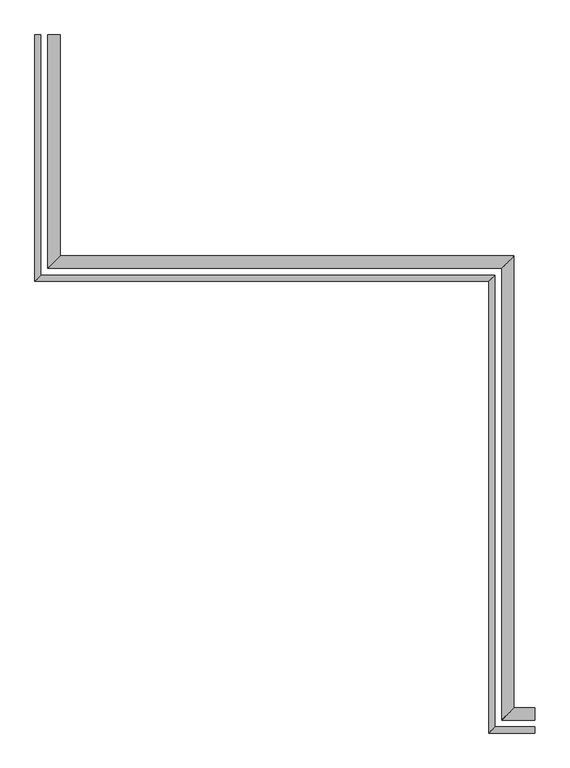
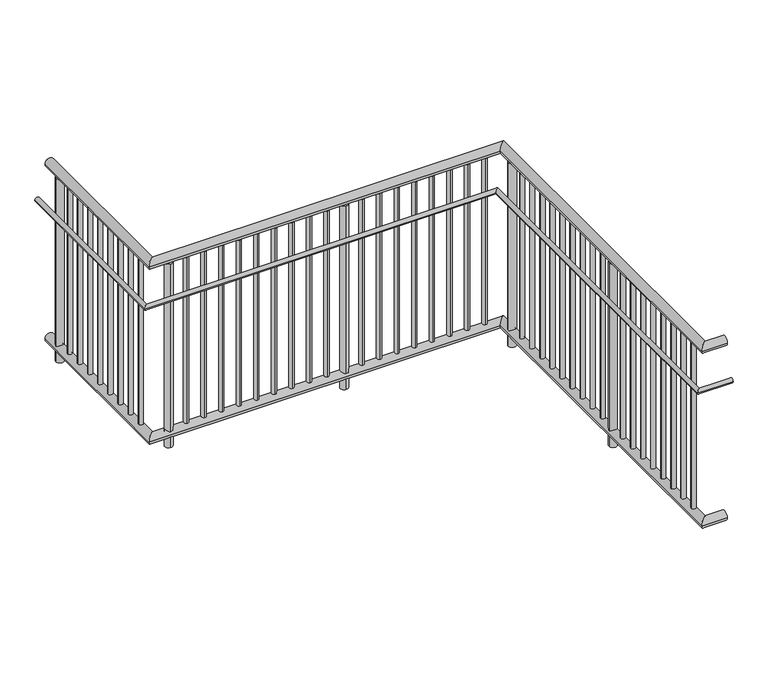
"""IFC4 building model written with IfcOpenShell, lengths in millimetres: railing geometry."""

import ifcopenshell
import ifcopenshell.guid

model = None  # the IFC model being written
_history = None  # IfcOwnerHistory: only IFC2X3 demands one
_inside = {}  # id of a spatial element -> (the spatial element, [elements in it])
_under = {}  # id of a project, library or spatial element -> (it, [spatial elements below it])
_declared = {}  # id of a project -> (the project, [libraries it declares])
_typed = {}  # id of a type object -> (the type object, [elements of that type])
_made_of = {}  # id of a material, layer set ... -> (it, [elements and type objects made of it])


def new_model(schema):
    """Start an empty IFC model of exactly this schema.

    Asked for "IFC4X3", IfcOpenShell would pick the latest addendum, in which some entities
    have other attributes; the version numbers below select the first issue.
    IFC2X3 requires an IfcOwnerHistory on every rooted entity: one is made here for all.
    """
    global model, _history
    if schema == "IFC4X3":
        model = ifcopenshell.file(schema_version=(4, 3, 0, 0))
    else:
        model = ifcopenshell.file(schema=schema)
    _inside.clear()
    _under.clear()
    _declared.clear()
    _typed.clear()
    _made_of.clear()
    _history = None
    if model.schema == "IFC2X3":
        org = make("IfcOrganization", Name="unknown")
        user = make(
            "IfcPersonAndOrganization",
            ThePerson=make("IfcPerson", FamilyName="unknown"),
            TheOrganization=org,
        )
        app = make(
            "IfcApplication",
            ApplicationDeveloper=org,
            Version="unknown",
            ApplicationFullName="unknown",
            ApplicationIdentifier="unknown",
        )
        _history = make(
            "IfcOwnerHistory",
            OwningUser=user,
            OwningApplication=app,
            ChangeAction="ADDED",
            CreationDate=0,
        )
    return model


def make(cls, **values):
    """One entity of the class cls with the attributes given. An attribute that is None is left unset."""
    return model.create_entity(
        cls, **{name: value for name, value in values.items() if value is not None}
    )


def rooted(cls, **values):
    """An entity with a GlobalId (a new one), such as an element, a storey or a relation."""
    return make(cls, GlobalId=ifcopenshell.guid.new(), OwnerHistory=_history, **values)


def si_unit(unit_type, name, prefix=None):
    """IfcSIUnit, for example si_unit("LENGTHUNIT", "METRE", prefix="MILLI")."""
    return make("IfcSIUnit", UnitType=unit_type, Prefix=prefix, Name=name)


def assignment(units):
    """IfcUnitAssignment: the units of a project."""
    return None if units is None else make("IfcUnitAssignment", Units=units)


def point(xyz):
    """IfcCartesianPoint."""
    return None if xyz is None else make("IfcCartesianPoint", Coordinates=xyz)


def direction(xyz):
    """IfcDirection."""
    return None if xyz is None else make("IfcDirection", DirectionRatios=xyz)


def frame(location, z_axis=None, x_axis=None):
    """IfcAxis2Placement3D, a coordinate frame: its origin and axes. An axis left out is left unset."""
    return make(
        "IfcAxis2Placement3D",
        Location=point(location),
        Axis=direction(z_axis),
        RefDirection=direction(x_axis),
    )


def frame_2d(location, x_axis=None):
    """IfcAxis2Placement2D, a coordinate frame in the plane: its origin and x axis."""
    return make(
        "IfcAxis2Placement2D", Location=point(location), RefDirection=direction(x_axis)
    )


def origin():
    """The frame at (0, 0, 0) with its axes left unset."""
    return frame((0.0, 0.0, 0.0))


def place(relative_to, where):
    """IfcLocalPlacement: puts the frame where relative to a parent placement (None: the world)."""
    return make(
        "IfcLocalPlacement", PlacementRelTo=relative_to, RelativePlacement=where
    )


def context(
    kind, dimensions, precision=None, world=None, true_north=None, identifier=None
):
    """IfcGeometricRepresentationContext, for example the 3D "Model" context."""
    return make(
        "IfcGeometricRepresentationContext",
        ContextIdentifier=identifier,
        ContextType=kind,
        CoordinateSpaceDimension=dimensions,
        Precision=precision,
        WorldCoordinateSystem=world,
        TrueNorth=true_north,
    )


def project(units=None, contexts=None):
    """IfcProject with its units and contexts."""
    return rooted(
        "IfcProject",
        Name="project",
        RepresentationContexts=contexts,
        UnitsInContext=assignment(units),
    )


def spatial(cls, under=None, at=None, **own):
    """A site, building, storey or space (cls), placed at a placement, below another one or the project."""
    s = rooted(cls, ObjectPlacement=at, **own)
    if under is not None:
        _under.setdefault(under.id(), (under, []))[1].append(s)
    return s


def circle_curve(where, radius):
    """IfcCircle in the frame where."""
    return make("IfcCircle", Position=where, Radius=radius)


def ellipse_curve(where, semi_axis1, semi_axis2):
    """IfcEllipse in the frame where."""
    return make(
        "IfcEllipse", Position=where, SemiAxis1=semi_axis1, SemiAxis2=semi_axis2
    )


def trimmed(basis, trim1, trim2, sense, master):
    """IfcTrimmedCurve: the piece of a basis curve between two trims."""
    return make(
        "IfcTrimmedCurve",
        BasisCurve=basis,
        Trim1=trim1,
        Trim2=trim2,
        SenseAgreement=sense,
        MasterRepresentation=master,
    )


def segment(curve, same_sense, transition):
    """IfcCompositeCurveSegment."""
    return make(
        "IfcCompositeCurveSegment",
        Transition=transition,
        SameSense=same_sense,
        ParentCurve=curve,
    )


def composite_curve(segments, self_intersect=None):
    """IfcCompositeCurve: segments joined end to end."""
    return make("IfcCompositeCurve", Segments=segments, SelfIntersect=self_intersect)


def outline(outer, holes=None, kind="AREA"):
    """IfcArbitraryClosedProfileDef: a profile drawn as a closed curve; with holes, ...WithVoids."""
    if holes is None:
        return make("IfcArbitraryClosedProfileDef", ProfileType=kind, OuterCurve=outer)
    return make(
        "IfcArbitraryProfileDefWithVoids",
        ProfileType=kind,
        OuterCurve=outer,
        InnerCurves=holes,
    )


def extrude(swept, where, along, depth):
    """IfcExtrudedAreaSolid: the profile swept, set in the frame where, extruded along a direction by depth."""
    return make(
        "IfcExtrudedAreaSolid",
        SweptArea=swept,
        Position=where,
        ExtrudedDirection=direction(along),
        Depth=depth,
    )


def shape(context_of_items, identifier, shape_type, items):
    """IfcShapeRepresentation: the items that make up one representation, for example the "Body"."""
    return make(
        "IfcShapeRepresentation",
        ContextOfItems=context_of_items,
        RepresentationIdentifier=identifier,
        RepresentationType=shape_type,
        Items=items,
    )


def source(mapping_origin, context_of_items, identifier, shape_type, items):
    """IfcRepresentationMap: a shape defined once, which mapped items show again and again."""
    return make(
        "IfcRepresentationMap",
        MappingOrigin=mapping_origin,
        MappedRepresentation=shape(context_of_items, identifier, shape_type, items),
    )


def transform(
    local_origin,
    x_axis=None,
    y_axis=None,
    z_axis=None,
    scale=None,
    scale2=None,
    scale3=None,
    uniform=True,
):
    """IfcCartesianTransformationOperator3D, or its non-uniform kind. x_axis, y_axis, z_axis: its Axis1, 2, 3."""
    if uniform:
        return make(
            "IfcCartesianTransformationOperator3D",
            Axis1=direction(x_axis),
            Axis2=direction(y_axis),
            LocalOrigin=point(local_origin),
            Scale=scale,
            Axis3=direction(z_axis),
        )
    return make(
        "IfcCartesianTransformationOperator3DnonUniform",
        Axis1=direction(x_axis),
        Axis2=direction(y_axis),
        LocalOrigin=point(local_origin),
        Scale=scale,
        Axis3=direction(z_axis),
        Scale2=scale2,
        Scale3=scale3,
    )


def mapped(mapping_source, mapping_target):
    """IfcMappedItem: shows the shape of a source again, moved by a transform."""
    return make(
        "IfcMappedItem", MappingSource=mapping_source, MappingTarget=mapping_target
    )


def made_of(thing, what):
    """Note that an element or type object is made of a material, layer set ...; save() writes the relation."""
    if what is not None:
        _made_of.setdefault(what.id(), (what, []))[1].append(thing)
    return thing


def element(
    cls,
    number,
    at=None,
    inside=None,
    cuts=None,
    type_object=None,
    material=None,
    context=None,
    identifier="Body",
    shape_type=None,
    held_by="IfcProductDefinitionShape",
    body=None,
    shapes=None,
    **own,
):
    """One element of the class cls, such as IfcWall. Its Tag is "e" and its number.

    at: its placement. inside: the storey or other place that contains it. cuts: it is an
    opening in that element (IfcRelVoidsElement). A single representation is given by context,
    identifier, shape_type and body (its items); several are given by shapes. held_by: the class
    of the entity that holds the representations. save() writes the other relations.
    """
    e = rooted(cls, Tag="e%d" % number, ObjectPlacement=at, **own)
    if body is not None:
        shapes = [shape(context, identifier, shape_type, body)]
    if shapes is not None:
        e.Representation = make(held_by, Representations=shapes)
    if inside is not None:
        _inside.setdefault(inside.id(), (inside, []))[1].append(e)
    if cuts is not None:
        rooted(
            "IfcRelVoidsElement", RelatingBuildingElement=cuts, RelatedOpeningElement=e
        )
    if type_object is not None:
        _typed.setdefault(type_object.id(), (type_object, []))[1].append(e)
    return made_of(e, material)


def aggregate(whole, parts):
    """IfcRelAggregates: a whole, such as a stair, and the parts it consists of."""
    return rooted("IfcRelAggregates", RelatingObject=whole, RelatedObjects=parts)


def save(model, path):
    """Write the relations noted so far, then the file.

    IfcRelAggregates (storeys below a building ...), IfcRelContainedInSpatialStructure (elements
    in a storey), IfcRelDefinesByType, IfcRelAssociatesMaterial and IfcRelDeclares: one each for
    every whole, place, type object, material and project.
    """
    for whole, parts in _under.values():
        aggregate(whole, parts)
    for where, things in _inside.values():
        rooted(
            "IfcRelContainedInSpatialStructure",
            RelatedElements=things,
            RelatingStructure=where,
        )
    for kind, things in _typed.values():
        rooted("IfcRelDefinesByType", RelatedObjects=things, RelatingType=kind)
    for what, things in _made_of.values():
        rooted("IfcRelAssociatesMaterial", RelatedObjects=things, RelatingMaterial=what)
    for by, libraries in _declared.values():
        rooted("IfcRelDeclares", RelatingContext=by, RelatedDefinitions=libraries)
    model.write(path)


def plane_surface(at):
    """IfcPlane: the flat surface through the origin of the frame at, square to its z axis."""
    return make("IfcPlane", Position=at)


def cylinder_surface(at, radius):
    """IfcCylindricalSurface: all points at the distance radius from the z axis of the frame at."""
    return make("IfcCylindricalSurface", Position=at, Radius=radius)


def advanced_brep(points, edges, surfaces, faces):
    """IfcAdvancedBrep: a solid bounded by faces that lie on surfaces and meet in shared edges.

    An edge is (start, end): straight between two places in points (the first is 0);
    or (start, end, curve); or (start, end, curve, False) where it runs against its curve.
    A face is (place in surfaces, loops), or (place, loops, False) where it looks against
    its surface's normal. A loop lists edges by number (the first is 1), with a minus sign
    where the edge is run from its end to its start. The first loop is the outer one.
    """
    corners = [point(p) for p in points]
    vertices = [make("IfcVertexPoint", VertexGeometry=c) for c in corners]
    made = []
    for start, end, *more in edges:
        made.append(
            make(
                "IfcEdgeCurve",
                EdgeStart=vertices[start],
                EdgeEnd=vertices[end],
                EdgeGeometry=more[0] if more else make("IfcPolyline", Points=[corners[start], corners[end]]),
                SameSense=more[1] if len(more) > 1 else True,
            )
        )
    hull = []
    for where, loops, *sense in faces:
        bounds = []
        for j, loop in enumerate(loops):
            ring = [make("IfcOrientedEdge", EdgeElement=made[abs(k) - 1], Orientation=k > 0) for k in loop]
            bounds.append(
                make(
                    "IfcFaceOuterBound" if j == 0 else "IfcFaceBound",
                    Bound=make("IfcEdgeLoop", EdgeList=ring),
                    Orientation=True,
                )
            )
        hull.append(make("IfcAdvancedFace", Bounds=bounds, FaceSurface=surfaces[where], SameSense=sense[0] if sense else True))
    return make("IfcAdvancedBrep", Outer=make("IfcClosedShell", CfsFaces=hull))


def railing_76a26c40(model_context):
    return source(origin(), model_context, "Body", "SolidModel", [
        advanced_brep(
        [(655.125551, -901.0965465, 4474.6), (604.325551, -901.0965465, 4474.6), (655.125551, -1825.6965465, 4474.6), (604.325551, -1876.4965465, 4474.6), (2555.125551, -1825.6965465, 4474.6), (2504.325551, -1876.4965465, 4474.6), (2555.125551, -3715.6965465, 4474.6), (2504.325551, -3766.4965465, 4474.6), (2643.025551, -3715.6965465, 4474.6), (2643.025551, -3766.4965465, 4474.6)],
        [
            (0, 1, circle_curve(frame((629.725551, -901.0965465, 4474.6), z_axis=(0.0, 1.0, 0.0), x_axis=(-1.0, 0.0, 0.0)), 25.4)),
            (1, 0, circle_curve(frame((629.725551, -901.0965465, 4474.6), z_axis=(0.0, 1.0, 0.0), x_axis=(-1.0, 0.0, 0.0)), 25.4)),
            (0, 2),
            (2, 3, ellipse_curve(frame((629.725551, -1851.0965465, 4474.6), z_axis=(-0.7071067811865475, 0.7071067811865475, 0.0), x_axis=(0.7071067811865474, 0.7071067811865476, 0.0)), 35.9210245, 25.4)),
            (3, 1),
            (3, 2, ellipse_curve(frame((629.725551, -1851.0965465, 4474.6), z_axis=(-0.7071067811865475, 0.7071067811865475, 0.0), x_axis=(0.7071067811865474, 0.7071067811865476, 0.0)), 35.9210245, 25.4)),
            (2, 4),
            (4, 5, ellipse_curve(frame((2529.725551, -1851.0965465, 4474.6), z_axis=(-0.7071067811865475, 0.7071067811865475, 0.0), x_axis=(-0.7071067811865476, -0.7071067811865474, 0.0)), 35.9210245, 25.4)),
            (5, 3),
            (5, 4, ellipse_curve(frame((2529.725551, -1851.0965465, 4474.6), z_axis=(-0.7071067811865475, 0.7071067811865475, 0.0), x_axis=(-0.7071067811865476, -0.7071067811865474, 0.0)), 35.9210245, 25.4)),
            (4, 6),
            (6, 7, ellipse_curve(frame((2529.725551, -3741.0965465, 4474.6), z_axis=(-0.7071067811865475, 0.7071067811865475, 0.0), x_axis=(0.7071067811865474, 0.7071067811865476, 0.0)), 35.9210245, 25.4)),
            (7, 5),
            (7, 6, ellipse_curve(frame((2529.725551, -3741.0965465, 4474.6), z_axis=(-0.7071067811865475, 0.7071067811865475, 0.0), x_axis=(0.7071067811865474, 0.7071067811865476, 0.0)), 35.9210245, 25.4)),
            (8, 9, circle_curve(frame((2643.025551, -3741.0965465, 4474.6), z_axis=(1.0, 0.0, 0.0), x_axis=(0.0, -1.0, 0.0)), 25.4)),
            (9, 8, circle_curve(frame((2643.025551, -3741.0965465, 4474.6), z_axis=(1.0, 0.0, 0.0), x_axis=(0.0, -1.0, 0.0)), 25.4)),
            (6, 8),
            (9, 7),
        ],
        [
            plane_surface(frame((629.725551, -901.0965465, 4500.0), z_axis=(0.0, 1.0, 0.0), x_axis=(0.0, 0.0, -1.0))),
            cylinder_surface(frame((629.725551, -901.0965465, 4474.6), z_axis=(0.0, 1.0, 0.0), x_axis=(-1.0, 0.0, 0.0)), 25.4),
            cylinder_surface(frame((629.725551, -1851.0965465, 4474.6), z_axis=(-1.0, 0.0, 0.0), x_axis=(0.0, -1.0, 0.0)), 25.4),
            cylinder_surface(frame((2529.725551, -1851.0965465, 4474.6), z_axis=(0.0, 1.0, 0.0), x_axis=(-1.0, 0.0, 0.0)), 25.4),
            plane_surface(frame((2643.025551, -3741.0965465, 4500.0), z_axis=(1.0, 0.0, 0.0), x_axis=(0.0, 1.0, 0.0))),
            cylinder_surface(frame((2529.725551, -3741.0965465, 4474.6), z_axis=(-1.0, 0.0, 0.0), x_axis=(0.0, -1.0, 0.0)), 25.4),
        ],
        [
            (0, [[1, 2]]),
            (1, [[-1, 3, 4, 5]]),
            (1, [[-2, -5, 6, -3]]),
            (2, [[-4, 7, 8, 9]]),
            (2, [[-6, -9, 10, -7]]),
            (3, [[-8, 11, 12, 13]]),
            (3, [[-10, -13, 14, -11]]),
            (4, [[15, 16]]),
            (5, [[-12, 17, -16, 18]]),
            (5, [[-14, -18, -15, -17]]),
        ],
    ),
        advanced_brep(
        [(575.425551, -901.0965465, 4287.3), (550.025551, -901.0965465, 4287.3), (575.425551, -1905.3965465, 4287.3), (550.025551, -1930.7965465, 4287.3), (2475.425551, -1905.3965465, 4287.3), (2450.025551, -1930.7965465, 4287.3), (2475.425551, -3795.3965465, 4287.3), (2450.025551, -3820.7965465, 4287.3), (2643.025551, -3795.3965465, 4287.3), (2643.025551, -3820.7965465, 4287.3)],
        [
            (0, 1, circle_curve(frame((562.725551, -901.0965465, 4287.3), z_axis=(0.0, 1.0, 0.0), x_axis=(-1.0, 0.0, 0.0)), 12.7)),
            (1, 0, circle_curve(frame((562.725551, -901.0965465, 4287.3), z_axis=(0.0, 1.0, 0.0), x_axis=(-1.0, 0.0, 0.0)), 12.7)),
            (0, 2),
            (2, 3, ellipse_curve(frame((562.725551, -1918.0965465, 4287.3), z_axis=(-0.7071067811865475, 0.7071067811865475, 0.0), x_axis=(0.7071067811865474, 0.7071067811865476, 0.0)), 17.9605122, 12.7)),
            (3, 1),
            (3, 2, ellipse_curve(frame((562.725551, -1918.0965465, 4287.3), z_axis=(-0.7071067811865475, 0.7071067811865475, 0.0), x_axis=(0.7071067811865474, 0.7071067811865476, 0.0)), 17.9605122, 12.7)),
            (2, 4),
            (4, 5, ellipse_curve(frame((2462.725551, -1918.0965465, 4287.3), z_axis=(-0.7071067811865475, 0.7071067811865475, 0.0), x_axis=(-0.7071067811865476, -0.7071067811865474, 0.0)), 17.9605122, 12.7)),
            (5, 3),
            (5, 4, ellipse_curve(frame((2462.725551, -1918.0965465, 4287.3), z_axis=(-0.7071067811865475, 0.7071067811865475, 0.0), x_axis=(-0.7071067811865476, -0.7071067811865474, 0.0)), 17.9605122, 12.7)),
            (4, 6),
            (6, 7, ellipse_curve(frame((2462.725551, -3808.0965465, 4287.3), z_axis=(-0.7071067811865475, 0.7071067811865475, 0.0), x_axis=(0.7071067811865474, 0.7071067811865476, 0.0)), 17.9605122, 12.7)),
            (7, 5),
            (7, 6, ellipse_curve(frame((2462.725551, -3808.0965465, 4287.3), z_axis=(-0.7071067811865475, 0.7071067811865475, 0.0), x_axis=(0.7071067811865474, 0.7071067811865476, 0.0)), 17.9605122, 12.7)),
            (8, 9, circle_curve(frame((2643.025551, -3808.0965465, 4287.3), z_axis=(1.0, 0.0, 0.0), x_axis=(0.0, -1.0, 0.0)), 12.7)),
            (9, 8, circle_curve(frame((2643.025551, -3808.0965465, 4287.3), z_axis=(1.0, 0.0, 0.0), x_axis=(0.0, -1.0, 0.0)), 12.7)),
            (6, 8),
            (9, 7),
        ],
        [
            plane_surface(frame((562.725551, -901.0965465, 4300.0), z_axis=(0.0, 1.0, 0.0), x_axis=(0.0, 0.0, -1.0))),
            cylinder_surface(frame((562.725551, -901.0965465, 4287.3), z_axis=(0.0, 1.0, 0.0), x_axis=(-1.0, 0.0, 0.0)), 12.7),
            cylinder_surface(frame((562.725551, -1918.0965465, 4287.3), z_axis=(-1.0, 0.0, 0.0), x_axis=(0.0, -1.0, 0.0)), 12.7),
            cylinder_surface(frame((2462.725551, -1918.0965465, 4287.3), z_axis=(0.0, 1.0, 0.0), x_axis=(-1.0, 0.0, 0.0)), 12.7),
            plane_surface(frame((2643.025551, -3808.0965465, 4300.0), z_axis=(1.0, 0.0, 0.0), x_axis=(0.0, 1.0, 0.0))),
            cylinder_surface(frame((2462.725551, -3808.0965465, 4287.3), z_axis=(-1.0, 0.0, 0.0), x_axis=(0.0, -1.0, 0.0)), 12.7),
        ],
        [
            (0, [[1, 2]]),
            (1, [[-1, 3, 4, 5]]),
            (1, [[-2, -5, 6, -3]]),
            (2, [[-4, 7, 8, 9]]),
            (2, [[-6, -9, 10, -7]]),
            (3, [[-8, 11, 12, 13]]),
            (3, [[-10, -13, 14, -11]]),
            (4, [[15, 16]]),
            (5, [[-12, 17, -16, 18]]),
            (5, [[-14, -18, -15, -17]]),
        ],
    ),
        advanced_brep(
        [(655.125551, -901.0965465, 3474.6), (604.325551, -901.0965465, 3474.6), (655.125551, -1825.6965465, 3474.6), (604.325551, -1876.4965465, 3474.6), (2555.125551, -1825.6965465, 3474.6), (2504.325551, -1876.4965465, 3474.6), (2555.125551, -3715.6965465, 3474.6), (2504.325551, -3766.4965465, 3474.6), (2643.025551, -3715.6965465, 3474.6), (2643.025551, -3766.4965465, 3474.6)],
        [
            (0, 1, circle_curve(frame((629.725551, -901.0965465, 3474.6), z_axis=(0.0, 1.0, 0.0), x_axis=(-1.0, 0.0, 0.0)), 25.4)),
            (1, 0, circle_curve(frame((629.725551, -901.0965465, 3474.6), z_axis=(0.0, 1.0, 0.0), x_axis=(-1.0, 0.0, 0.0)), 25.4)),
            (0, 2),
            (2, 3, ellipse_curve(frame((629.725551, -1851.0965465, 3474.6), z_axis=(-0.7071067811865475, 0.7071067811865475, 0.0), x_axis=(0.7071067811865474, 0.7071067811865476, 0.0)), 35.9210245, 25.4)),
            (3, 1),
            (3, 2, ellipse_curve(frame((629.725551, -1851.0965465, 3474.6), z_axis=(-0.7071067811865475, 0.7071067811865475, 0.0), x_axis=(0.7071067811865474, 0.7071067811865476, 0.0)), 35.9210245, 25.4)),
            (2, 4),
            (4, 5, ellipse_curve(frame((2529.725551, -1851.0965465, 3474.6), z_axis=(-0.7071067811865475, 0.7071067811865475, 0.0), x_axis=(-0.7071067811865476, -0.7071067811865474, 0.0)), 35.9210245, 25.4)),
            (5, 3),
            (5, 4, ellipse_curve(frame((2529.725551, -1851.0965465, 3474.6), z_axis=(-0.7071067811865475, 0.7071067811865475, 0.0), x_axis=(-0.7071067811865476, -0.7071067811865474, 0.0)), 35.9210245, 25.4)),
            (4, 6),
            (6, 7, ellipse_curve(frame((2529.725551, -3741.0965465, 3474.6), z_axis=(-0.7071067811865475, 0.7071067811865475, 0.0), x_axis=(0.7071067811865474, 0.7071067811865476, 0.0)), 35.9210245, 25.4)),
            (7, 5),
            (7, 6, ellipse_curve(frame((2529.725551, -3741.0965465, 3474.6), z_axis=(-0.7071067811865475, 0.7071067811865475, 0.0), x_axis=(0.7071067811865474, 0.7071067811865476, 0.0)), 35.9210245, 25.4)),
            (8, 9, circle_curve(frame((2643.025551, -3741.0965465, 3474.6), z_axis=(1.0, 0.0, 0.0), x_axis=(0.0, -1.0, 0.0)), 25.4)),
            (9, 8, circle_curve(frame((2643.025551, -3741.0965465, 3474.6), z_axis=(1.0, 0.0, 0.0), x_axis=(0.0, -1.0, 0.0)), 25.4)),
            (6, 8),
            (9, 7),
        ],
        [
            plane_surface(frame((629.725551, -901.0965465, 3500.0), z_axis=(0.0, 1.0, 0.0), x_axis=(0.0, 0.0, -1.0))),
            cylinder_surface(frame((629.725551, -901.0965465, 3474.6), z_axis=(0.0, 1.0, 0.0), x_axis=(-1.0, 0.0, 0.0)), 25.4),
            cylinder_surface(frame((629.725551, -1851.0965465, 3474.6), z_axis=(-1.0, 0.0, 0.0), x_axis=(0.0, -1.0, 0.0)), 25.4),
            cylinder_surface(frame((2529.725551, -1851.0965465, 3474.6), z_axis=(0.0, 1.0, 0.0), x_axis=(-1.0, 0.0, 0.0)), 25.4),
            plane_surface(frame((2643.025551, -3741.0965465, 3500.0), z_axis=(1.0, 0.0, 0.0), x_axis=(0.0, 1.0, 0.0))),
            cylinder_surface(frame((2529.725551, -3741.0965465, 3474.6), z_axis=(-1.0, 0.0, 0.0), x_axis=(0.0, -1.0, 0.0)), 25.4),
        ],
        [
            (0, [[1, 2]]),
            (1, [[-1, 3, 4, 5]]),
            (1, [[-2, -5, 6, -3]]),
            (2, [[-4, 7, 8, 9]]),
            (2, [[-6, -9, 10, -7]]),
            (3, [[-8, 11, 12, 13]]),
            (3, [[-10, -13, 14, -11]]),
            (4, [[15, 16]]),
            (5, [[-12, 17, -16, 18]]),
            (5, [[-14, -18, -15, -17]]),
        ],
    ),
        extrude(outline(composite_curve([segment(trimmed(circle_curve(frame_2d((2529.725551, -3646.5965465)), 12.5), [point((2542.225551, -3646.5965465))], [point((2517.225551, -3646.5965465))], False, "CARTESIAN"), True, "CONTINUOUS"), segment(trimmed(circle_curve(frame_2d((2529.725551, -3646.5965465)), 12.5), [point((2517.225551, -3646.5965465))], [point((2542.225551, -3646.5965465))], False, "CARTESIAN"), True, "CONTINUOUS")], self_intersect=False)), frame((0.0, 0.0, 3500.0), z_axis=(0.0, 0.0, 1.0), x_axis=(1.0, 0.0, 0.0)), (0.0, 0.0, 1.0), 949.2),
        extrude(outline(composite_curve([segment(trimmed(circle_curve(frame_2d((2529.725551, -3552.0965465)), 12.5), [point((2542.225551, -3552.0965465))], [point((2517.225551, -3552.0965465))], False, "CARTESIAN"), True, "CONTINUOUS"), segment(trimmed(circle_curve(frame_2d((2529.725551, -3552.0965465)), 12.5), [point((2517.225551, -3552.0965465))], [point((2542.225551, -3552.0965465))], False, "CARTESIAN"), True, "CONTINUOUS")], self_intersect=False)), frame((0.0, 0.0, 3500.0), z_axis=(0.0, 0.0, 1.0), x_axis=(1.0, 0.0, 0.0)), (0.0, 0.0, 1.0), 949.2),
        extrude(outline(composite_curve([segment(trimmed(circle_curve(frame_2d((2529.725551, -3457.5965465)), 12.5), [point((2542.225551, -3457.5965465))], [point((2517.225551, -3457.5965465))], False, "CARTESIAN"), True, "CONTINUOUS"), segment(trimmed(circle_curve(frame_2d((2529.725551, -3457.5965465)), 12.5), [point((2517.225551, -3457.5965465))], [point((2542.225551, -3457.5965465))], False, "CARTESIAN"), True, "CONTINUOUS")], self_intersect=False)), frame((0.0, 0.0, 3500.0), z_axis=(0.0, 0.0, 1.0), x_axis=(1.0, 0.0, 0.0)), (0.0, 0.0, 1.0), 949.2),
        extrude(outline(composite_curve([segment(trimmed(circle_curve(frame_2d((2529.725551, -3363.0965465)), 12.5), [point((2542.225551, -3363.0965465))], [point((2517.225551, -3363.0965465))], False, "CARTESIAN"), True, "CONTINUOUS"), segment(trimmed(circle_curve(frame_2d((2529.725551, -3363.0965465)), 12.5), [point((2517.225551, -3363.0965465))], [point((2542.225551, -3363.0965465))], False, "CARTESIAN"), True, "CONTINUOUS")], self_intersect=False)), frame((0.0, 0.0, 3500.0), z_axis=(0.0, 0.0, 1.0), x_axis=(1.0, 0.0, 0.0)), (0.0, 0.0, 1.0), 949.2),
        extrude(outline(composite_curve([segment(trimmed(circle_curve(frame_2d((2529.725551, -3268.5965465)), 12.5), [point((2542.225551, -3268.5965465))], [point((2517.225551, -3268.5965465))], False, "CARTESIAN"), True, "CONTINUOUS"), segment(trimmed(circle_curve(frame_2d((2529.725551, -3268.5965465)), 12.5), [point((2517.225551, -3268.5965465))], [point((2542.225551, -3268.5965465))], False, "CARTESIAN"), True, "CONTINUOUS")], self_intersect=False)), frame((0.0, 0.0, 3500.0), z_axis=(0.0, 0.0, 1.0), x_axis=(1.0, 0.0, 0.0)), (0.0, 0.0, 1.0), 949.2),
        extrude(outline(composite_curve([segment(trimmed(circle_curve(frame_2d((2529.725551, -3174.0965465)), 12.5), [point((2542.225551, -3174.0965465))], [point((2517.225551, -3174.0965465))], False, "CARTESIAN"), True, "CONTINUOUS"), segment(trimmed(circle_curve(frame_2d((2529.725551, -3174.0965465)), 12.5), [point((2517.225551, -3174.0965465))], [point((2542.225551, -3174.0965465))], False, "CARTESIAN"), True, "CONTINUOUS")], self_intersect=False)), frame((0.0, 0.0, 3500.0), z_axis=(0.0, 0.0, 1.0), x_axis=(1.0, 0.0, 0.0)), (0.0, 0.0, 1.0), 949.2),
        extrude(outline(composite_curve([segment(trimmed(circle_curve(frame_2d((2529.725551, -3079.5965465)), 12.5), [point((2542.225551, -3079.5965465))], [point((2517.225551, -3079.5965465))], False, "CARTESIAN"), True, "CONTINUOUS"), segment(trimmed(circle_curve(frame_2d((2529.725551, -3079.5965465)), 12.5), [point((2517.225551, -3079.5965465))], [point((2542.225551, -3079.5965465))], False, "CARTESIAN"), True, "CONTINUOUS")], self_intersect=False)), frame((0.0, 0.0, 3500.0), z_axis=(0.0, 0.0, 1.0), x_axis=(1.0, 0.0, 0.0)), (0.0, 0.0, 1.0), 949.2),
        extrude(outline(composite_curve([segment(trimmed(circle_curve(frame_2d((2529.725551, -2985.0965465)), 12.5), [point((2542.225551, -2985.0965465))], [point((2517.225551, -2985.0965465))], False, "CARTESIAN"), True, "CONTINUOUS"), segment(trimmed(circle_curve(frame_2d((2529.725551, -2985.0965465)), 12.5), [point((2517.225551, -2985.0965465))], [point((2542.225551, -2985.0965465))], False, "CARTESIAN"), True, "CONTINUOUS")], self_intersect=False)), frame((0.0, 0.0, 3500.0), z_axis=(0.0, 0.0, 1.0), x_axis=(1.0, 0.0, 0.0)), (0.0, 0.0, 1.0), 949.2),
        extrude(outline(composite_curve([segment(trimmed(circle_curve(frame_2d((2529.725551, -2890.5965465)), 21.0), [point((2550.725551, -2890.5965465))], [point((2508.725551, -2890.5965465))], False, "CARTESIAN"), True, "CONTINUOUS"), segment(trimmed(circle_curve(frame_2d((2529.725551, -2890.5965465)), 21.0), [point((2508.725551, -2890.5965465))], [point((2550.725551, -2890.5965465))], False, "CARTESIAN"), True, "CONTINUOUS")], self_intersect=False)), frame((0.0, 0.0, 3400.0), z_axis=(0.0, 0.0, 1.0), x_axis=(1.0, 0.0, 0.0)), (0.0, 0.0, 1.0), 1049.2),
        extrude(outline(composite_curve([segment(trimmed(circle_curve(frame_2d((2529.725551, -2796.0965465)), 12.5), [point((2542.225551, -2796.0965465))], [point((2517.225551, -2796.0965465))], False, "CARTESIAN"), True, "CONTINUOUS"), segment(trimmed(circle_curve(frame_2d((2529.725551, -2796.0965465)), 12.5), [point((2517.225551, -2796.0965465))], [point((2542.225551, -2796.0965465))], False, "CARTESIAN"), True, "CONTINUOUS")], self_intersect=False)), frame((0.0, 0.0, 3500.0), z_axis=(0.0, 0.0, 1.0), x_axis=(1.0, 0.0, 0.0)), (0.0, 0.0, 1.0), 949.2),
        extrude(outline(composite_curve([segment(trimmed(circle_curve(frame_2d((2529.725551, -2701.5965465)), 12.5), [point((2542.225551, -2701.5965465))], [point((2517.225551, -2701.5965465))], False, "CARTESIAN"), True, "CONTINUOUS"), segment(trimmed(circle_curve(frame_2d((2529.725551, -2701.5965465)), 12.5), [point((2517.225551, -2701.5965465))], [point((2542.225551, -2701.5965465))], False, "CARTESIAN"), True, "CONTINUOUS")], self_intersect=False)), frame((0.0, 0.0, 3500.0), z_axis=(0.0, 0.0, 1.0), x_axis=(1.0, 0.0, 0.0)), (0.0, 0.0, 1.0), 949.2),
        extrude(outline(composite_curve([segment(trimmed(circle_curve(frame_2d((2529.725551, -2607.0965465)), 12.5), [point((2542.225551, -2607.0965465))], [point((2517.225551, -2607.0965465))], False, "CARTESIAN"), True, "CONTINUOUS"), segment(trimmed(circle_curve(frame_2d((2529.725551, -2607.0965465)), 12.5), [point((2517.225551, -2607.0965465))], [point((2542.225551, -2607.0965465))], False, "CARTESIAN"), True, "CONTINUOUS")], self_intersect=False)), frame((0.0, 0.0, 3500.0), z_axis=(0.0, 0.0, 1.0), x_axis=(1.0, 0.0, 0.0)), (0.0, 0.0, 1.0), 949.2),
        extrude(outline(composite_curve([segment(trimmed(circle_curve(frame_2d((2529.725551, -2512.5965465)), 12.5), [point((2542.225551, -2512.5965465))], [point((2517.225551, -2512.5965465))], False, "CARTESIAN"), True, "CONTINUOUS"), segment(trimmed(circle_curve(frame_2d((2529.725551, -2512.5965465)), 12.5), [point((2517.225551, -2512.5965465))], [point((2542.225551, -2512.5965465))], False, "CARTESIAN"), True, "CONTINUOUS")], self_intersect=False)), frame((0.0, 0.0, 3500.0), z_axis=(0.0, 0.0, 1.0), x_axis=(1.0, 0.0, 0.0)), (0.0, 0.0, 1.0), 949.2),
        extrude(outline(composite_curve([segment(trimmed(circle_curve(frame_2d((2529.725551, -2418.0965465)), 12.5), [point((2542.225551, -2418.0965465))], [point((2517.225551, -2418.0965465))], False, "CARTESIAN"), True, "CONTINUOUS"), segment(trimmed(circle_curve(frame_2d((2529.725551, -2418.0965465)), 12.5), [point((2517.225551, -2418.0965465))], [point((2542.225551, -2418.0965465))], False, "CARTESIAN"), True, "CONTINUOUS")], self_intersect=False)), frame((0.0, 0.0, 3500.0), z_axis=(0.0, 0.0, 1.0), x_axis=(1.0, 0.0, 0.0)), (0.0, 0.0, 1.0), 949.2),
        extrude(outline(composite_curve([segment(trimmed(circle_curve(frame_2d((2529.725551, -2323.5965465)), 12.5), [point((2542.225551, -2323.5965465))], [point((2517.225551, -2323.5965465))], False, "CARTESIAN"), True, "CONTINUOUS"), segment(trimmed(circle_curve(frame_2d((2529.725551, -2323.5965465)), 12.5), [point((2517.225551, -2323.5965465))], [point((2542.225551, -2323.5965465))], False, "CARTESIAN"), True, "CONTINUOUS")], self_intersect=False)), frame((0.0, 0.0, 3500.0), z_axis=(0.0, 0.0, 1.0), x_axis=(1.0, 0.0, 0.0)), (0.0, 0.0, 1.0), 949.2),
        extrude(outline(composite_curve([segment(trimmed(circle_curve(frame_2d((2529.725551, -2229.0965465)), 12.5), [point((2542.225551, -2229.0965465))], [point((2517.225551, -2229.0965465))], False, "CARTESIAN"), True, "CONTINUOUS"), segment(trimmed(circle_curve(frame_2d((2529.725551, -2229.0965465)), 12.5), [point((2517.225551, -2229.0965465))], [point((2542.225551, -2229.0965465))], False, "CARTESIAN"), True, "CONTINUOUS")], self_intersect=False)), frame((0.0, 0.0, 3500.0), z_axis=(0.0, 0.0, 1.0), x_axis=(1.0, 0.0, 0.0)), (0.0, 0.0, 1.0), 949.2),
        extrude(outline(composite_curve([segment(trimmed(circle_curve(frame_2d((2529.725551, -2134.5965465)), 12.5), [point((2542.225551, -2134.5965465))], [point((2517.225551, -2134.5965465))], False, "CARTESIAN"), True, "CONTINUOUS"), segment(trimmed(circle_curve(frame_2d((2529.725551, -2134.5965465)), 12.5), [point((2517.225551, -2134.5965465))], [point((2542.225551, -2134.5965465))], False, "CARTESIAN"), True, "CONTINUOUS")], self_intersect=False)), frame((0.0, 0.0, 3500.0), z_axis=(0.0, 0.0, 1.0), x_axis=(1.0, 0.0, 0.0)), (0.0, 0.0, 1.0), 949.2),
        extrude(outline(composite_curve([segment(trimmed(circle_curve(frame_2d((2529.725551, -2040.0965465)), 12.5), [point((2542.225551, -2040.0965465))], [point((2517.225551, -2040.0965465))], False, "CARTESIAN"), True, "CONTINUOUS"), segment(trimmed(circle_curve(frame_2d((2529.725551, -2040.0965465)), 12.5), [point((2517.225551, -2040.0965465))], [point((2542.225551, -2040.0965465))], False, "CARTESIAN"), True, "CONTINUOUS")], self_intersect=False)), frame((0.0, 0.0, 3500.0), z_axis=(0.0, 0.0, 1.0), x_axis=(1.0, 0.0, 0.0)), (0.0, 0.0, 1.0), 949.2),
        extrude(outline(composite_curve([segment(trimmed(circle_curve(frame_2d((2529.725551, -1945.5965465)), 21.0), [point((2550.725551, -1945.5965465))], [point((2508.725551, -1945.5965465))], False, "CARTESIAN"), True, "CONTINUOUS"), segment(trimmed(circle_curve(frame_2d((2529.725551, -1945.5965465)), 21.0), [point((2508.725551, -1945.5965465))], [point((2550.725551, -1945.5965465))], False, "CARTESIAN"), True, "CONTINUOUS")], self_intersect=False)), frame((0.0, 0.0, 3400.0), z_axis=(0.0, 0.0, 1.0), x_axis=(1.0, 0.0, 0.0)), (0.0, 0.0, 1.0), 1049.2),
        extrude(outline(composite_curve([segment(trimmed(circle_curve(frame_2d((2434.725551, -1851.0965465)), 12.5), [point((2434.725551, -1838.5965465))], [point((2434.725551, -1863.5965465))], False, "CARTESIAN"), True, "CONTINUOUS"), segment(trimmed(circle_curve(frame_2d((2434.725551, -1851.0965465)), 12.5), [point((2434.725551, -1863.5965465))], [point((2434.725551, -1838.5965465))], False, "CARTESIAN"), True, "CONTINUOUS")], self_intersect=False)), frame((0.0, 0.0, 3500.0), z_axis=(0.0, 0.0, 1.0), x_axis=(1.0, 0.0, 0.0)), (0.0, 0.0, 1.0), 949.2),
        extrude(outline(composite_curve([segment(trimmed(circle_curve(frame_2d((2339.725551, -1851.0965465)), 12.5), [point((2339.725551, -1838.5965465))], [point((2339.725551, -1863.5965465))], False, "CARTESIAN"), True, "CONTINUOUS"), segment(trimmed(circle_curve(frame_2d((2339.725551, -1851.0965465)), 12.5), [point((2339.725551, -1863.5965465))], [point((2339.725551, -1838.5965465))], False, "CARTESIAN"), True, "CONTINUOUS")], self_intersect=False)), frame((0.0, 0.0, 3500.0), z_axis=(0.0, 0.0, 1.0), x_axis=(1.0, 0.0, 0.0)), (0.0, 0.0, 1.0), 949.2),
        extrude(outline(composite_curve([segment(trimmed(circle_curve(frame_2d((2244.725551, -1851.0965465)), 12.5), [point((2244.725551, -1838.5965465))], [point((2244.725551, -1863.5965465))], False, "CARTESIAN"), True, "CONTINUOUS"), segment(trimmed(circle_curve(frame_2d((2244.725551, -1851.0965465)), 12.5), [point((2244.725551, -1863.5965465))], [point((2244.725551, -1838.5965465))], False, "CARTESIAN"), True, "CONTINUOUS")], self_intersect=False)), frame((0.0, 0.0, 3500.0), z_axis=(0.0, 0.0, 1.0), x_axis=(1.0, 0.0, 0.0)), (0.0, 0.0, 1.0), 949.2),
        extrude(outline(composite_curve([segment(trimmed(circle_curve(frame_2d((2149.725551, -1851.0965465)), 12.5), [point((2149.725551, -1838.5965465))], [point((2149.725551, -1863.5965465))], False, "CARTESIAN"), True, "CONTINUOUS"), segment(trimmed(circle_curve(frame_2d((2149.725551, -1851.0965465)), 12.5), [point((2149.725551, -1863.5965465))], [point((2149.725551, -1838.5965465))], False, "CARTESIAN"), True, "CONTINUOUS")], self_intersect=False)), frame((0.0, 0.0, 3500.0), z_axis=(0.0, 0.0, 1.0), x_axis=(1.0, 0.0, 0.0)), (0.0, 0.0, 1.0), 949.2),
        extrude(outline(composite_curve([segment(trimmed(circle_curve(frame_2d((2054.725551, -1851.0965465)), 12.5), [point((2054.725551, -1838.5965465))], [point((2054.725551, -1863.5965465))], False, "CARTESIAN"), True, "CONTINUOUS"), segment(trimmed(circle_curve(frame_2d((2054.725551, -1851.0965465)), 12.5), [point((2054.725551, -1863.5965465))], [point((2054.725551, -1838.5965465))], False, "CARTESIAN"), True, "CONTINUOUS")], self_intersect=False)), frame((0.0, 0.0, 3500.0), z_axis=(0.0, 0.0, 1.0), x_axis=(1.0, 0.0, 0.0)), (0.0, 0.0, 1.0), 949.2),
        extrude(outline(composite_curve([segment(trimmed(circle_curve(frame_2d((1959.725551, -1851.0965465)), 12.5), [point((1959.725551, -1838.5965465))], [point((1959.725551, -1863.5965465))], False, "CARTESIAN"), True, "CONTINUOUS"), segment(trimmed(circle_curve(frame_2d((1959.725551, -1851.0965465)), 12.5), [point((1959.725551, -1863.5965465))], [point((1959.725551, -1838.5965465))], False, "CARTESIAN"), True, "CONTINUOUS")], self_intersect=False)), frame((0.0, 0.0, 3500.0), z_axis=(0.0, 0.0, 1.0), x_axis=(1.0, 0.0, 0.0)), (0.0, 0.0, 1.0), 949.2),
        extrude(outline(composite_curve([segment(trimmed(circle_curve(frame_2d((1864.725551, -1851.0965465)), 12.5), [point((1864.725551, -1838.5965465))], [point((1864.725551, -1863.5965465))], False, "CARTESIAN"), True, "CONTINUOUS"), segment(trimmed(circle_curve(frame_2d((1864.725551, -1851.0965465)), 12.5), [point((1864.725551, -1863.5965465))], [point((1864.725551, -1838.5965465))], False, "CARTESIAN"), True, "CONTINUOUS")], self_intersect=False)), frame((0.0, 0.0, 3500.0), z_axis=(0.0, 0.0, 1.0), x_axis=(1.0, 0.0, 0.0)), (0.0, 0.0, 1.0), 949.2),
        extrude(outline(composite_curve([segment(trimmed(circle_curve(frame_2d((1769.725551, -1851.0965465)), 12.5), [point((1769.725551, -1838.5965465))], [point((1769.725551, -1863.5965465))], False, "CARTESIAN"), True, "CONTINUOUS"), segment(trimmed(circle_curve(frame_2d((1769.725551, -1851.0965465)), 12.5), [point((1769.725551, -1863.5965465))], [point((1769.725551, -1838.5965465))], False, "CARTESIAN"), True, "CONTINUOUS")], self_intersect=False)), frame((0.0, 0.0, 3500.0), z_axis=(0.0, 0.0, 1.0), x_axis=(1.0, 0.0, 0.0)), (0.0, 0.0, 1.0), 949.2),
        extrude(outline(composite_curve([segment(trimmed(circle_curve(frame_2d((1674.725551, -1851.0965465)), 21.0), [point((1674.725551, -1830.0965465))], [point((1674.725551, -1872.0965465))], False, "CARTESIAN"), True, "CONTINUOUS"), segment(trimmed(circle_curve(frame_2d((1674.725551, -1851.0965465)), 21.0), [point((1674.725551, -1872.0965465))], [point((1674.725551, -1830.0965465))], False, "CARTESIAN"), True, "CONTINUOUS")], self_intersect=False)), frame((0.0, 0.0, 3400.0), z_axis=(0.0, 0.0, 1.0), x_axis=(1.0, 0.0, 0.0)), (0.0, 0.0, 1.0), 1049.2),
        extrude(outline(composite_curve([segment(trimmed(circle_curve(frame_2d((1579.725551, -1851.0965465)), 12.5), [point((1579.725551, -1838.5965465))], [point((1579.725551, -1863.5965465))], False, "CARTESIAN"), True, "CONTINUOUS"), segment(trimmed(circle_curve(frame_2d((1579.725551, -1851.0965465)), 12.5), [point((1579.725551, -1863.5965465))], [point((1579.725551, -1838.5965465))], False, "CARTESIAN"), True, "CONTINUOUS")], self_intersect=False)), frame((0.0, 0.0, 3500.0), z_axis=(0.0, 0.0, 1.0), x_axis=(1.0, 0.0, 0.0)), (0.0, 0.0, 1.0), 949.2),
        extrude(outline(composite_curve([segment(trimmed(circle_curve(frame_2d((1484.725551, -1851.0965465)), 12.5), [point((1484.725551, -1838.5965465))], [point((1484.725551, -1863.5965465))], False, "CARTESIAN"), True, "CONTINUOUS"), segment(trimmed(circle_curve(frame_2d((1484.725551, -1851.0965465)), 12.5), [point((1484.725551, -1863.5965465))], [point((1484.725551, -1838.5965465))], False, "CARTESIAN"), True, "CONTINUOUS")], self_intersect=False)), frame((0.0, 0.0, 3500.0), z_axis=(0.0, 0.0, 1.0), x_axis=(1.0, 0.0, 0.0)), (0.0, 0.0, 1.0), 949.2),
        extrude(outline(composite_curve([segment(trimmed(circle_curve(frame_2d((1389.725551, -1851.0965465)), 12.5), [point((1389.725551, -1838.5965465))], [point((1389.725551, -1863.5965465))], False, "CARTESIAN"), True, "CONTINUOUS"), segment(trimmed(circle_curve(frame_2d((1389.725551, -1851.0965465)), 12.5), [point((1389.725551, -1863.5965465))], [point((1389.725551, -1838.5965465))], False, "CARTESIAN"), True, "CONTINUOUS")], self_intersect=False)), frame((0.0, 0.0, 3500.0), z_axis=(0.0, 0.0, 1.0), x_axis=(1.0, 0.0, 0.0)), (0.0, 0.0, 1.0), 949.2),
        extrude(outline(composite_curve([segment(trimmed(circle_curve(frame_2d((1294.725551, -1851.0965465)), 12.5), [point((1294.725551, -1838.5965465))], [point((1294.725551, -1863.5965465))], False, "CARTESIAN"), True, "CONTINUOUS"), segment(trimmed(circle_curve(frame_2d((1294.725551, -1851.0965465)), 12.5), [point((1294.725551, -1863.5965465))], [point((1294.725551, -1838.5965465))], False, "CARTESIAN"), True, "CONTINUOUS")], self_intersect=False)), frame((0.0, 0.0, 3500.0), z_axis=(0.0, 0.0, 1.0), x_axis=(1.0, 0.0, 0.0)), (0.0, 0.0, 1.0), 949.2),
        extrude(outline(composite_curve([segment(trimmed(circle_curve(frame_2d((1199.725551, -1851.0965465)), 12.5), [point((1199.725551, -1838.5965465))], [point((1199.725551, -1863.5965465))], False, "CARTESIAN"), True, "CONTINUOUS"), segment(trimmed(circle_curve(frame_2d((1199.725551, -1851.0965465)), 12.5), [point((1199.725551, -1863.5965465))], [point((1199.725551, -1838.5965465))], False, "CARTESIAN"), True, "CONTINUOUS")], self_intersect=False)), frame((0.0, 0.0, 3500.0), z_axis=(0.0, 0.0, 1.0), x_axis=(1.0, 0.0, 0.0)), (0.0, 0.0, 1.0), 949.2),
        extrude(outline(composite_curve([segment(trimmed(circle_curve(frame_2d((1104.725551, -1851.0965465)), 12.5), [point((1104.725551, -1838.5965465))], [point((1104.725551, -1863.5965465))], False, "CARTESIAN"), True, "CONTINUOUS"), segment(trimmed(circle_curve(frame_2d((1104.725551, -1851.0965465)), 12.5), [point((1104.725551, -1863.5965465))], [point((1104.725551, -1838.5965465))], False, "CARTESIAN"), True, "CONTINUOUS")], self_intersect=False)), frame((0.0, 0.0, 3500.0), z_axis=(0.0, 0.0, 1.0), x_axis=(1.0, 0.0, 0.0)), (0.0, 0.0, 1.0), 949.2),
        extrude(outline(composite_curve([segment(trimmed(circle_curve(frame_2d((1009.725551, -1851.0965465)), 12.5), [point((1009.725551, -1838.5965465))], [point((1009.725551, -1863.5965465))], False, "CARTESIAN"), True, "CONTINUOUS"), segment(trimmed(circle_curve(frame_2d((1009.725551, -1851.0965465)), 12.5), [point((1009.725551, -1863.5965465))], [point((1009.725551, -1838.5965465))], False, "CARTESIAN"), True, "CONTINUOUS")], self_intersect=False)), frame((0.0, 0.0, 3500.0), z_axis=(0.0, 0.0, 1.0), x_axis=(1.0, 0.0, 0.0)), (0.0, 0.0, 1.0), 949.2),
        extrude(outline(composite_curve([segment(trimmed(circle_curve(frame_2d((914.725551, -1851.0965465)), 12.5), [point((914.725551, -1838.5965465))], [point((914.725551, -1863.5965465))], False, "CARTESIAN"), True, "CONTINUOUS"), segment(trimmed(circle_curve(frame_2d((914.725551, -1851.0965465)), 12.5), [point((914.725551, -1863.5965465))], [point((914.725551, -1838.5965465))], False, "CARTESIAN"), True, "CONTINUOUS")], self_intersect=False)), frame((0.0, 0.0, 3500.0), z_axis=(0.0, 0.0, 1.0), x_axis=(1.0, 0.0, 0.0)), (0.0, 0.0, 1.0), 949.2),
        extrude(outline(composite_curve([segment(trimmed(circle_curve(frame_2d((819.725551, -1851.0965465)), 12.5), [point((819.725551, -1838.5965465))], [point((819.725551, -1863.5965465))], False, "CARTESIAN"), True, "CONTINUOUS"), segment(trimmed(circle_curve(frame_2d((819.725551, -1851.0965465)), 12.5), [point((819.725551, -1863.5965465))], [point((819.725551, -1838.5965465))], False, "CARTESIAN"), True, "CONTINUOUS")], self_intersect=False)), frame((0.0, 0.0, 3500.0), z_axis=(0.0, 0.0, 1.0), x_axis=(1.0, 0.0, 0.0)), (0.0, 0.0, 1.0), 949.2),
        extrude(outline(composite_curve([segment(trimmed(circle_curve(frame_2d((724.725551, -1851.0965465)), 21.0), [point((724.725551, -1830.0965465))], [point((724.725551, -1872.0965465))], False, "CARTESIAN"), True, "CONTINUOUS"), segment(trimmed(circle_curve(frame_2d((724.725551, -1851.0965465)), 21.0), [point((724.725551, -1872.0965465))], [point((724.725551, -1830.0965465))], False, "CARTESIAN"), True, "CONTINUOUS")], self_intersect=False)), frame((0.0, 0.0, 3400.0), z_axis=(0.0, 0.0, 1.0), x_axis=(1.0, 0.0, 0.0)), (0.0, 0.0, 1.0), 1049.2),
        extrude(outline(composite_curve([segment(trimmed(circle_curve(frame_2d((629.725551, -1756.0965465)), 12.5), [point((642.225551, -1756.0965465))], [point((617.225551, -1756.0965465))], False, "CARTESIAN"), True, "CONTINUOUS"), segment(trimmed(circle_curve(frame_2d((629.725551, -1756.0965465)), 12.5), [point((617.225551, -1756.0965465))], [point((642.225551, -1756.0965465))], False, "CARTESIAN"), True, "CONTINUOUS")], self_intersect=False)), frame((0.0, 0.0, 3500.0), z_axis=(0.0, 0.0, 1.0), x_axis=(1.0, 0.0, 0.0)), (0.0, 0.0, 1.0), 949.2),
        extrude(outline(composite_curve([segment(trimmed(circle_curve(frame_2d((629.725551, -1661.0965465)), 12.5), [point((642.225551, -1661.0965465))], [point((617.225551, -1661.0965465))], False, "CARTESIAN"), True, "CONTINUOUS"), segment(trimmed(circle_curve(frame_2d((629.725551, -1661.0965465)), 12.5), [point((617.225551, -1661.0965465))], [point((642.225551, -1661.0965465))], False, "CARTESIAN"), True, "CONTINUOUS")], self_intersect=False)), frame((0.0, 0.0, 3500.0), z_axis=(0.0, 0.0, 1.0), x_axis=(1.0, 0.0, 0.0)), (0.0, 0.0, 1.0), 949.2),
        extrude(outline(composite_curve([segment(trimmed(circle_curve(frame_2d((629.725551, -1566.0965465)), 12.5), [point((642.225551, -1566.0965465))], [point((617.225551, -1566.0965465))], False, "CARTESIAN"), True, "CONTINUOUS"), segment(trimmed(circle_curve(frame_2d((629.725551, -1566.0965465)), 12.5), [point((617.225551, -1566.0965465))], [point((642.225551, -1566.0965465))], False, "CARTESIAN"), True, "CONTINUOUS")], self_intersect=False)), frame((0.0, 0.0, 3500.0), z_axis=(0.0, 0.0, 1.0), x_axis=(1.0, 0.0, 0.0)), (0.0, 0.0, 1.0), 949.2),
        extrude(outline(composite_curve([segment(trimmed(circle_curve(frame_2d((629.725551, -1471.0965465)), 12.5), [point((642.225551, -1471.0965465))], [point((617.225551, -1471.0965465))], False, "CARTESIAN"), True, "CONTINUOUS"), segment(trimmed(circle_curve(frame_2d((629.725551, -1471.0965465)), 12.5), [point((617.225551, -1471.0965465))], [point((642.225551, -1471.0965465))], False, "CARTESIAN"), True, "CONTINUOUS")], self_intersect=False)), frame((0.0, 0.0, 3500.0), z_axis=(0.0, 0.0, 1.0), x_axis=(1.0, 0.0, 0.0)), (0.0, 0.0, 1.0), 949.2),
        extrude(outline(composite_curve([segment(trimmed(circle_curve(frame_2d((629.725551, -1376.0965465)), 12.5), [point((642.225551, -1376.0965465))], [point((617.225551, -1376.0965465))], False, "CARTESIAN"), True, "CONTINUOUS"), segment(trimmed(circle_curve(frame_2d((629.725551, -1376.0965465)), 12.5), [point((617.225551, -1376.0965465))], [point((642.225551, -1376.0965465))], False, "CARTESIAN"), True, "CONTINUOUS")], self_intersect=False)), frame((0.0, 0.0, 3500.0), z_axis=(0.0, 0.0, 1.0), x_axis=(1.0, 0.0, 0.0)), (0.0, 0.0, 1.0), 949.2),
        extrude(outline(composite_curve([segment(trimmed(circle_curve(frame_2d((629.725551, -1281.0965465)), 12.5), [point((642.225551, -1281.0965465))], [point((617.225551, -1281.0965465))], False, "CARTESIAN"), True, "CONTINUOUS"), segment(trimmed(circle_curve(frame_2d((629.725551, -1281.0965465)), 12.5), [point((617.225551, -1281.0965465))], [point((642.225551, -1281.0965465))], False, "CARTESIAN"), True, "CONTINUOUS")], self_intersect=False)), frame((0.0, 0.0, 3500.0), z_axis=(0.0, 0.0, 1.0), x_axis=(1.0, 0.0, 0.0)), (0.0, 0.0, 1.0), 949.2),
        extrude(outline(composite_curve([segment(trimmed(circle_curve(frame_2d((629.725551, -1186.0965465)), 12.5), [point((642.225551, -1186.0965465))], [point((617.225551, -1186.0965465))], False, "CARTESIAN"), True, "CONTINUOUS"), segment(trimmed(circle_curve(frame_2d((629.725551, -1186.0965465)), 12.5), [point((617.225551, -1186.0965465))], [point((642.225551, -1186.0965465))], False, "CARTESIAN"), True, "CONTINUOUS")], self_intersect=False)), frame((0.0, 0.0, 3500.0), z_axis=(0.0, 0.0, 1.0), x_axis=(1.0, 0.0, 0.0)), (0.0, 0.0, 1.0), 949.2),
        extrude(outline(composite_curve([segment(trimmed(circle_curve(frame_2d((629.725551, -1091.0965465)), 12.5), [point((642.225551, -1091.0965465))], [point((617.225551, -1091.0965465))], False, "CARTESIAN"), True, "CONTINUOUS"), segment(trimmed(circle_curve(frame_2d((629.725551, -1091.0965465)), 12.5), [point((617.225551, -1091.0965465))], [point((642.225551, -1091.0965465))], False, "CARTESIAN"), True, "CONTINUOUS")], self_intersect=False)), frame((0.0, 0.0, 3500.0), z_axis=(0.0, 0.0, 1.0), x_axis=(1.0, 0.0, 0.0)), (0.0, 0.0, 1.0), 949.2),
        extrude(outline(composite_curve([segment(trimmed(circle_curve(frame_2d((629.725551, -996.0965465)), 21.0), [point((650.725551, -996.0965465))], [point((608.725551, -996.0965465))], False, "CARTESIAN"), True, "CONTINUOUS"), segment(trimmed(circle_curve(frame_2d((629.725551, -996.0965465)), 21.0), [point((608.725551, -996.0965465))], [point((650.725551, -996.0965465))], False, "CARTESIAN"), True, "CONTINUOUS")], self_intersect=False)), frame((0.0, 0.0, 3400.0), z_axis=(0.0, 0.0, 1.0), x_axis=(1.0, 0.0, 0.0)), (0.0, 0.0, 1.0), 1049.2),
    ])


if __name__ == "__main__":
    model = new_model("IFC4")
    model_context = context("Model", 3, world=origin())
    ifc_project = project(units=[si_unit("LENGTHUNIT", "METRE", prefix="MILLI")], contexts=[model_context])
    site = spatial("IfcSite", under=ifc_project)
    building = spatial("IfcBuilding", under=site)
    placement = place(None, origin())
    railing_shape = railing_76a26c40(model_context)
    element("IfcRailing", 1, at=placement, inside=building, context=model_context, shape_type="MappedRepresentation", body=[
        mapped(railing_shape, transform((0.0, 0.0, 0.0), x_axis=(1.0, 0.0, 0.0), y_axis=(0.0, 1.0, 0.0), z_axis=(0.0, 0.0, 1.0))),
    ])
    save(model, "model.ifc")

# Revit data of these elements
# Element 1 (IfcRailing)
#   Materials on its faces: "Ferro - Pintura Esmalte"
# Materials
#   "Ferro - Pintura Esmalte": class "Pintura", colour RGB 255 255 255, transparency 0, Cost = 0
